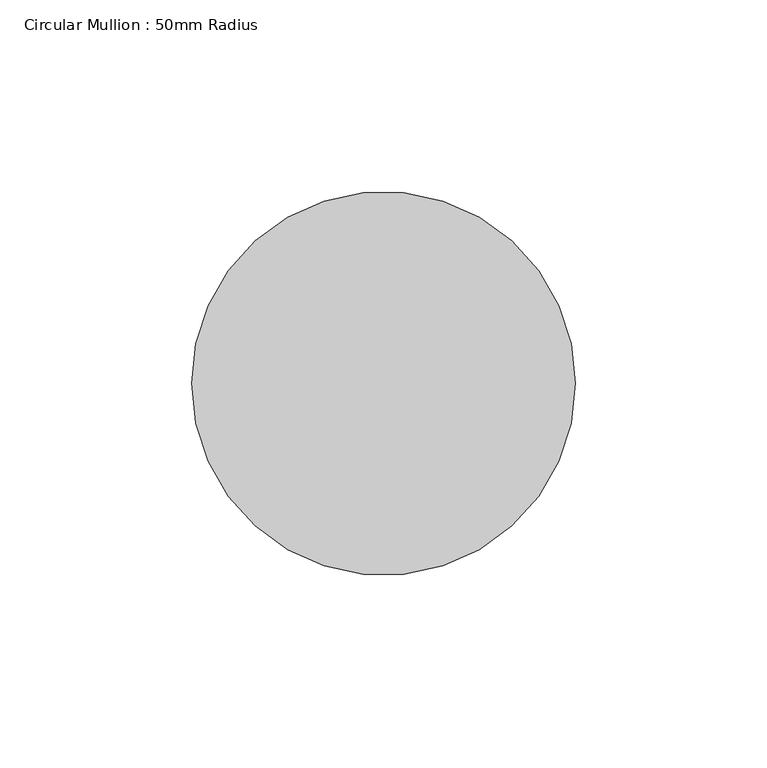
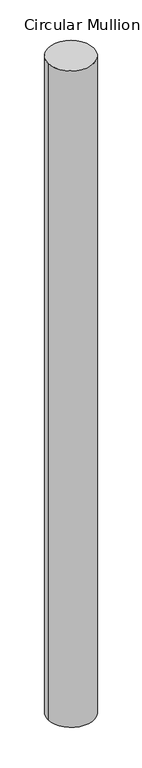
"""IFC4 building model written with IfcOpenShell, lengths in millimetres: member geometry, Circular Mullion : 50mm Radius."""

from ifc_helpers import new_model, si_unit, point, frame, origin, origin_2d, place, context, project, spatial, circle_curve, trimmed, segment, composite_curve, outline, extrude, source, transform, mapped, element, save


def circular_mullion_50mm_radius_3c4289b6(model_context):
    return source(origin(), model_context, "Body", "SweptSolid", [
        extrude(outline(composite_curve([segment(trimmed(circle_curve(origin_2d(), 50.0), [point((50.0, 0.0))], [point((-50.0, 0.0))], False, "CARTESIAN"), True, "CONTINUOUS"), segment(trimmed(circle_curve(origin_2d(), 50.0), [point((-50.0, 0.0))], [point((50.0, 0.0))], False, "CARTESIAN"), True, "CONTINUOUS")], self_intersect=False)), frame((0.0, 0.0, -1509.3539091), z_axis=(0.0, 0.0, 1.0), x_axis=(1.0, 0.0, 0.0)), (0.0, 0.0, 1.0), 1509.3539091),
    ])


if __name__ == "__main__":
    model = new_model("IFC4")
    model_context = context("Model", 3, world=origin())
    ifc_project = project(units=[si_unit("LENGTHUNIT", "METRE", prefix="MILLI")], contexts=[model_context])
    site = spatial("IfcSite", under=ifc_project)
    building = spatial("IfcBuilding", under=site)
    placement = place(None, origin())
    circular_mullion_50mm_radius_shape = circular_mullion_50mm_radius_3c4289b6(model_context)
    element("IfcMember", 1, ObjectType="Circular Mullion : 50mm Radius", at=placement, inside=building, context=model_context, shape_type="MappedRepresentation", body=[
        mapped(circular_mullion_50mm_radius_shape, transform((0.0, 0.0, 0.0), x_axis=(1.0, 0.0, 0.0), y_axis=(0.0, 1.0, 0.0), z_axis=(0.0, 0.0, 1.0))),
    ])
    save(model, "model.ifc")

# Revit data of these elements
# Type "Circular Mullion : 50mm Radius"
#   built-in parameter 1007350 = 0.164042 (stored number, unit not read)
# Element 1 (IfcMember, "Circular Mullion : 50mm Radius")
#   Materials on its faces: "Aluminium"
# Materials
#   "Aluminium": class "Metal", colour RGB 247 247 247, transparency 0, Description = "Aluminium 6061", Cost = 0
